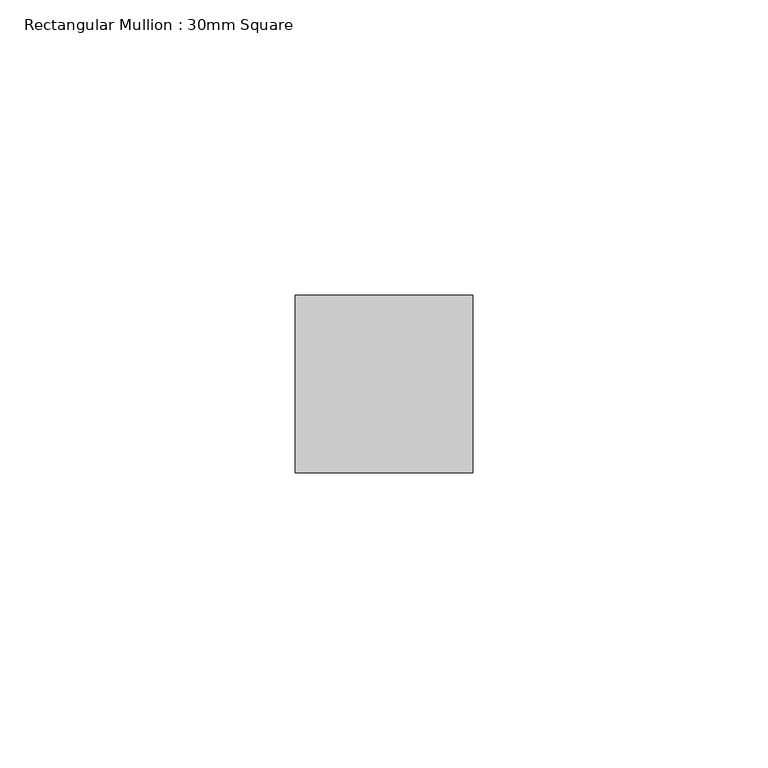
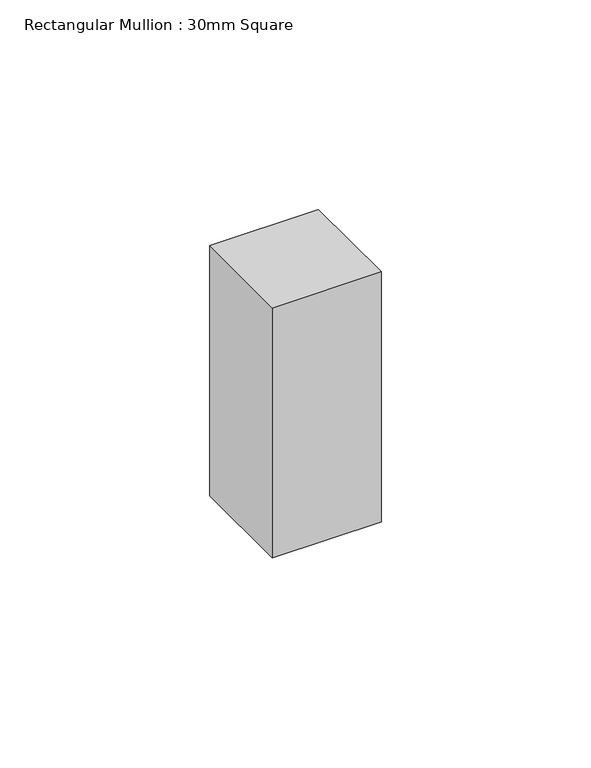
"""IFC4 building model written with IfcOpenShell, lengths in millimetres: member geometry, Rectangular Mullion : 30mm Square."""

from ifc_helpers import new_model, si_unit, frame, origin, place, context, project, spatial, polyline, outline, extrude, source, transform, mapped, element, save


def rectangular_mullion_30mm_square_b1eb862f(model_context):
    return source(origin(), model_context, "Body", "SweptSolid", [
        extrude(outline(polyline([(15.0, 15.0), (15.0, -15.0), (-15.0, -15.0), (-15.0, 15.0), (15.0, 15.0)])), frame((0.0, 0.0, -72.9386178), z_axis=(0.0, 0.0, 1.0), x_axis=(1.0, 0.0, 0.0)), (0.0, 0.0, 1.0), 72.9386178),
    ])


if __name__ == "__main__":
    model = new_model("IFC4")
    model_context = context("Model", 3, world=origin())
    ifc_project = project(units=[si_unit("LENGTHUNIT", "METRE", prefix="MILLI")], contexts=[model_context])
    site = spatial("IfcSite", under=ifc_project)
    building = spatial("IfcBuilding", under=site)
    placement = place(None, origin())
    rectangular_mullion_30mm_square_shape = rectangular_mullion_30mm_square_b1eb862f(model_context)
    element("IfcMember", 1, ObjectType="Rectangular Mullion : 30mm Square", at=placement, inside=building, context=model_context, shape_type="MappedRepresentation", body=[
        mapped(rectangular_mullion_30mm_square_shape, transform((0.0, 0.0, 0.0), x_axis=(1.0, 0.0, 0.0), y_axis=(0.0, 1.0, 0.0), z_axis=(0.0, 0.0, 1.0))),
    ])
    save(model, "model.ifc")

# Revit data of these elements
# Type "Rectangular Mullion : 30mm Square"
#   built-in parameter 1007304 = 0.0984252 (stored number, unit not read)
#   built-in parameter 1007301 = 0.0492126 (stored number, unit not read)
#   built-in parameter 1007300 = 0.0492126 (stored number, unit not read)
# Element 1 (IfcMember, "Rectangular Mullion : 30mm Square")
#   Materials on its faces: "Aluminum"
# Materials
#   "Aluminum": class "Metal", colour RGB 244 244 244, transparency 0, Description = "Aluminum 6061", Cost = 0
